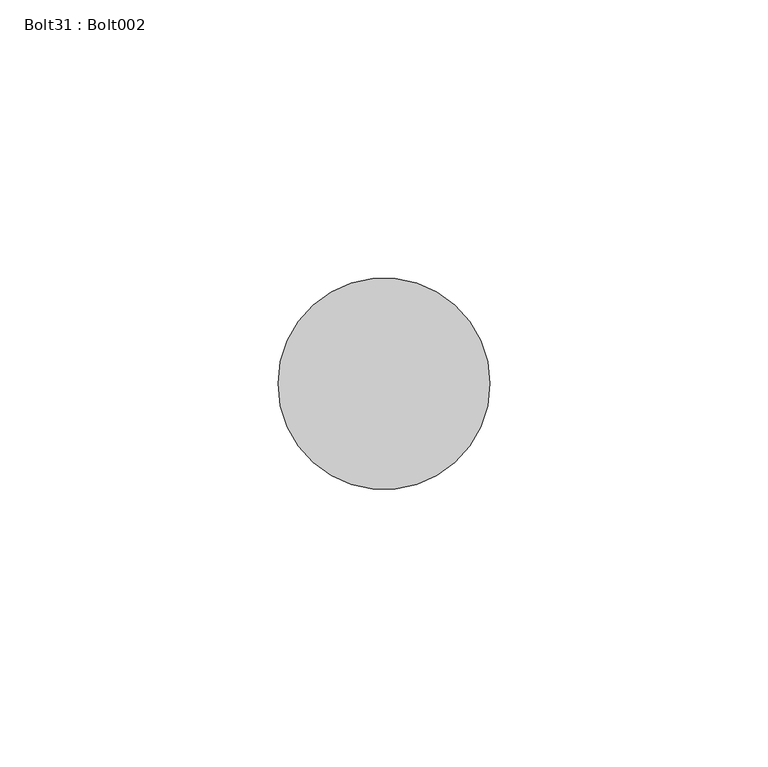
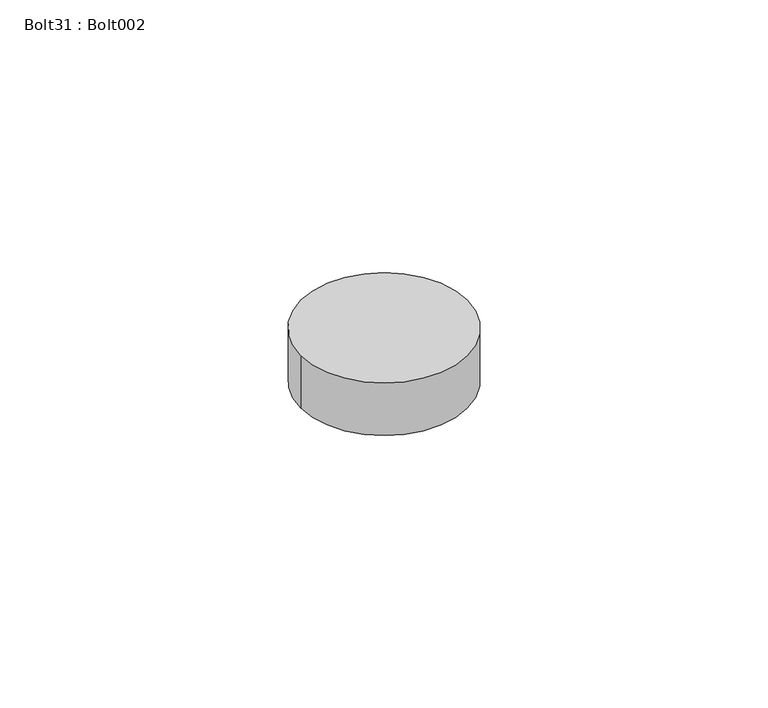
"""IFC4 building model written with IfcOpenShell, lengths in millimetres: proxy geometry, Bolt31 : Bolt002."""

import ifcopenshell
import ifcopenshell.guid

model = None  # the IFC model being written
_history = None  # IfcOwnerHistory: only IFC2X3 demands one
_inside = {}  # id of a spatial element -> (the spatial element, [elements in it])
_under = {}  # id of a project, library or spatial element -> (it, [spatial elements below it])
_declared = {}  # id of a project -> (the project, [libraries it declares])
_typed = {}  # id of a type object -> (the type object, [elements of that type])
_made_of = {}  # id of a material, layer set ... -> (it, [elements and type objects made of it])


def new_model(schema):
    """Start an empty IFC model of exactly this schema.

    Asked for "IFC4X3", IfcOpenShell would pick the latest addendum, in which some entities
    have other attributes; the version numbers below select the first issue.
    IFC2X3 requires an IfcOwnerHistory on every rooted entity: one is made here for all.
    """
    global model, _history
    if schema == "IFC4X3":
        model = ifcopenshell.file(schema_version=(4, 3, 0, 0))
    else:
        model = ifcopenshell.file(schema=schema)
    _inside.clear()
    _under.clear()
    _declared.clear()
    _typed.clear()
    _made_of.clear()
    _history = None
    if model.schema == "IFC2X3":
        org = make("IfcOrganization", Name="unknown")
        user = make(
            "IfcPersonAndOrganization",
            ThePerson=make("IfcPerson", FamilyName="unknown"),
            TheOrganization=org,
        )
        app = make(
            "IfcApplication",
            ApplicationDeveloper=org,
            Version="unknown",
            ApplicationFullName="unknown",
            ApplicationIdentifier="unknown",
        )
        _history = make(
            "IfcOwnerHistory",
            OwningUser=user,
            OwningApplication=app,
            ChangeAction="ADDED",
            CreationDate=0,
        )
    return model


def make(cls, **values):
    """One entity of the class cls with the attributes given. An attribute that is None is left unset."""
    return model.create_entity(
        cls, **{name: value for name, value in values.items() if value is not None}
    )


def rooted(cls, **values):
    """An entity with a GlobalId (a new one), such as an element, a storey or a relation."""
    return make(cls, GlobalId=ifcopenshell.guid.new(), OwnerHistory=_history, **values)


def si_unit(unit_type, name, prefix=None):
    """IfcSIUnit, for example si_unit("LENGTHUNIT", "METRE", prefix="MILLI")."""
    return make("IfcSIUnit", UnitType=unit_type, Prefix=prefix, Name=name)


def assignment(units):
    """IfcUnitAssignment: the units of a project."""
    return None if units is None else make("IfcUnitAssignment", Units=units)


def point(xyz):
    """IfcCartesianPoint."""
    return None if xyz is None else make("IfcCartesianPoint", Coordinates=xyz)


def direction(xyz):
    """IfcDirection."""
    return None if xyz is None else make("IfcDirection", DirectionRatios=xyz)


def frame(location, z_axis=None, x_axis=None):
    """IfcAxis2Placement3D, a coordinate frame: its origin and axes. An axis left out is left unset."""
    return make(
        "IfcAxis2Placement3D",
        Location=point(location),
        Axis=direction(z_axis),
        RefDirection=direction(x_axis),
    )


def frame_2d(location, x_axis=None):
    """IfcAxis2Placement2D, a coordinate frame in the plane: its origin and x axis."""
    return make(
        "IfcAxis2Placement2D", Location=point(location), RefDirection=direction(x_axis)
    )


def origin():
    """The frame at (0, 0, 0) with its axes left unset."""
    return frame((0.0, 0.0, 0.0))


def place(relative_to, where):
    """IfcLocalPlacement: puts the frame where relative to a parent placement (None: the world)."""
    return make(
        "IfcLocalPlacement", PlacementRelTo=relative_to, RelativePlacement=where
    )


def context(
    kind, dimensions, precision=None, world=None, true_north=None, identifier=None
):
    """IfcGeometricRepresentationContext, for example the 3D "Model" context."""
    return make(
        "IfcGeometricRepresentationContext",
        ContextIdentifier=identifier,
        ContextType=kind,
        CoordinateSpaceDimension=dimensions,
        Precision=precision,
        WorldCoordinateSystem=world,
        TrueNorth=true_north,
    )


def project(units=None, contexts=None):
    """IfcProject with its units and contexts."""
    return rooted(
        "IfcProject",
        Name="project",
        RepresentationContexts=contexts,
        UnitsInContext=assignment(units),
    )


def spatial(cls, under=None, at=None, **own):
    """A site, building, storey or space (cls), placed at a placement, below another one or the project."""
    s = rooted(cls, ObjectPlacement=at, **own)
    if under is not None:
        _under.setdefault(under.id(), (under, []))[1].append(s)
    return s


def circle_curve(where, radius):
    """IfcCircle in the frame where."""
    return make("IfcCircle", Position=where, Radius=radius)


def trimmed(basis, trim1, trim2, sense, master):
    """IfcTrimmedCurve: the piece of a basis curve between two trims."""
    return make(
        "IfcTrimmedCurve",
        BasisCurve=basis,
        Trim1=trim1,
        Trim2=trim2,
        SenseAgreement=sense,
        MasterRepresentation=master,
    )


def segment(curve, same_sense, transition):
    """IfcCompositeCurveSegment."""
    return make(
        "IfcCompositeCurveSegment",
        Transition=transition,
        SameSense=same_sense,
        ParentCurve=curve,
    )


def composite_curve(segments, self_intersect=None):
    """IfcCompositeCurve: segments joined end to end."""
    return make("IfcCompositeCurve", Segments=segments, SelfIntersect=self_intersect)


def outline(outer, holes=None, kind="AREA"):
    """IfcArbitraryClosedProfileDef: a profile drawn as a closed curve; with holes, ...WithVoids."""
    if holes is None:
        return make("IfcArbitraryClosedProfileDef", ProfileType=kind, OuterCurve=outer)
    return make(
        "IfcArbitraryProfileDefWithVoids",
        ProfileType=kind,
        OuterCurve=outer,
        InnerCurves=holes,
    )


def extrude(swept, where, along, depth):
    """IfcExtrudedAreaSolid: the profile swept, set in the frame where, extruded along a direction by depth."""
    return make(
        "IfcExtrudedAreaSolid",
        SweptArea=swept,
        Position=where,
        ExtrudedDirection=direction(along),
        Depth=depth,
    )


def shape(context_of_items, identifier, shape_type, items):
    """IfcShapeRepresentation: the items that make up one representation, for example the "Body"."""
    return make(
        "IfcShapeRepresentation",
        ContextOfItems=context_of_items,
        RepresentationIdentifier=identifier,
        RepresentationType=shape_type,
        Items=items,
    )


def source(mapping_origin, context_of_items, identifier, shape_type, items):
    """IfcRepresentationMap: a shape defined once, which mapped items show again and again."""
    return make(
        "IfcRepresentationMap",
        MappingOrigin=mapping_origin,
        MappedRepresentation=shape(context_of_items, identifier, shape_type, items),
    )


def transform(
    local_origin,
    x_axis=None,
    y_axis=None,
    z_axis=None,
    scale=None,
    scale2=None,
    scale3=None,
    uniform=True,
):
    """IfcCartesianTransformationOperator3D, or its non-uniform kind. x_axis, y_axis, z_axis: its Axis1, 2, 3."""
    if uniform:
        return make(
            "IfcCartesianTransformationOperator3D",
            Axis1=direction(x_axis),
            Axis2=direction(y_axis),
            LocalOrigin=point(local_origin),
            Scale=scale,
            Axis3=direction(z_axis),
        )
    return make(
        "IfcCartesianTransformationOperator3DnonUniform",
        Axis1=direction(x_axis),
        Axis2=direction(y_axis),
        LocalOrigin=point(local_origin),
        Scale=scale,
        Axis3=direction(z_axis),
        Scale2=scale2,
        Scale3=scale3,
    )


def mapped(mapping_source, mapping_target):
    """IfcMappedItem: shows the shape of a source again, moved by a transform."""
    return make(
        "IfcMappedItem", MappingSource=mapping_source, MappingTarget=mapping_target
    )


def made_of(thing, what):
    """Note that an element or type object is made of a material, layer set ...; save() writes the relation."""
    if what is not None:
        _made_of.setdefault(what.id(), (what, []))[1].append(thing)
    return thing


def element(
    cls,
    number,
    at=None,
    inside=None,
    cuts=None,
    type_object=None,
    material=None,
    context=None,
    identifier="Body",
    shape_type=None,
    held_by="IfcProductDefinitionShape",
    body=None,
    shapes=None,
    **own,
):
    """One element of the class cls, such as IfcWall. Its Tag is "e" and its number.

    at: its placement. inside: the storey or other place that contains it. cuts: it is an
    opening in that element (IfcRelVoidsElement). A single representation is given by context,
    identifier, shape_type and body (its items); several are given by shapes. held_by: the class
    of the entity that holds the representations. save() writes the other relations.
    """
    e = rooted(cls, Tag="e%d" % number, ObjectPlacement=at, **own)
    if body is not None:
        shapes = [shape(context, identifier, shape_type, body)]
    if shapes is not None:
        e.Representation = make(held_by, Representations=shapes)
    if inside is not None:
        _inside.setdefault(inside.id(), (inside, []))[1].append(e)
    if cuts is not None:
        rooted(
            "IfcRelVoidsElement", RelatingBuildingElement=cuts, RelatedOpeningElement=e
        )
    if type_object is not None:
        _typed.setdefault(type_object.id(), (type_object, []))[1].append(e)
    return made_of(e, material)


def aggregate(whole, parts):
    """IfcRelAggregates: a whole, such as a stair, and the parts it consists of."""
    return rooted("IfcRelAggregates", RelatingObject=whole, RelatedObjects=parts)


def save(model, path):
    """Write the relations noted so far, then the file.

    IfcRelAggregates (storeys below a building ...), IfcRelContainedInSpatialStructure (elements
    in a storey), IfcRelDefinesByType, IfcRelAssociatesMaterial and IfcRelDeclares: one each for
    every whole, place, type object, material and project.
    """
    for whole, parts in _under.values():
        aggregate(whole, parts)
    for where, things in _inside.values():
        rooted(
            "IfcRelContainedInSpatialStructure",
            RelatedElements=things,
            RelatingStructure=where,
        )
    for kind, things in _typed.values():
        rooted("IfcRelDefinesByType", RelatedObjects=things, RelatingType=kind)
    for what, things in _made_of.values():
        rooted("IfcRelAssociatesMaterial", RelatedObjects=things, RelatingMaterial=what)
    for by, libraries in _declared.values():
        rooted("IfcRelDeclares", RelatingContext=by, RelatedDefinitions=libraries)
    model.write(path)


def bolt31_bolt002_fd3bdce4(model_context):
    return source(origin(), model_context, "Body", "SweptSolid", [
        extrude(outline(composite_curve([segment(trimmed(circle_curve(frame_2d((5062.3346014, 1998.1882072)), 19.05), [point((5081.3846014, 1998.1882072))], [point((5043.2846014, 1998.1882072))], False, "CARTESIAN"), True, "CONTINUOUS"), segment(trimmed(circle_curve(frame_2d((5062.3346014, 1998.1882072)), 19.05), [point((5043.2846014, 1998.1882072))], [point((5081.3846014, 1998.1882072))], False, "CARTESIAN"), True, "CONTINUOUS")], self_intersect=False)), frame((0.0, 0.0, 36709.0959962), z_axis=(0.0, 0.0, 1.0), x_axis=(1.0, 0.0, 0.0)), (0.0, 0.0, 1.0), 12.7),
    ])


if __name__ == "__main__":
    model = new_model("IFC4")
    model_context = context("Model", 3, world=origin())
    ifc_project = project(units=[si_unit("LENGTHUNIT", "METRE", prefix="MILLI")], contexts=[model_context])
    site = spatial("IfcSite", under=ifc_project)
    building = spatial("IfcBuilding", under=site)
    placement = place(None, origin())
    bolt31_bolt002_shape = bolt31_bolt002_fd3bdce4(model_context)
    element("IfcBuildingElementProxy", 1, Name="Bolt31 : Bolt002", ObjectType="Bolt31 : Bolt002", at=placement, inside=building, context=model_context, shape_type="MappedRepresentation", body=[
        mapped(bolt31_bolt002_shape, transform((0.0, 0.0, 0.0), x_axis=(1.0, 0.0, 0.0), y_axis=(0.0, 1.0, 0.0), z_axis=(0.0, 0.0, 1.0))),
    ])
    save(model, "model.ifc")

# Revit data of these elements
# Type "Bolt31 : Bolt002"
#   NameOverride = "Bolt002"
# Element 1 (IfcBuildingElementProxy, "Bolt31 : Bolt002")
#   Materials on its faces: "STEEL ANGLE AND ANCHOR BOLT (SEE STRUCT. DWGS)"
# Materials
#   "STEEL ANGLE AND ANCHOR BOLT (SEE STRUCT. DWGS)": class "Unassigned", colour RGB 128 128 128, transparency 0, Cost = 0
